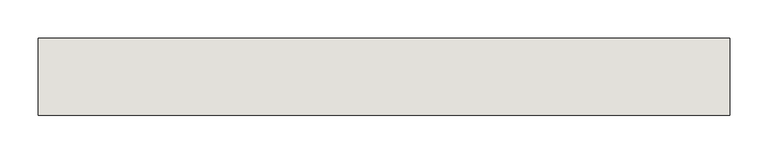
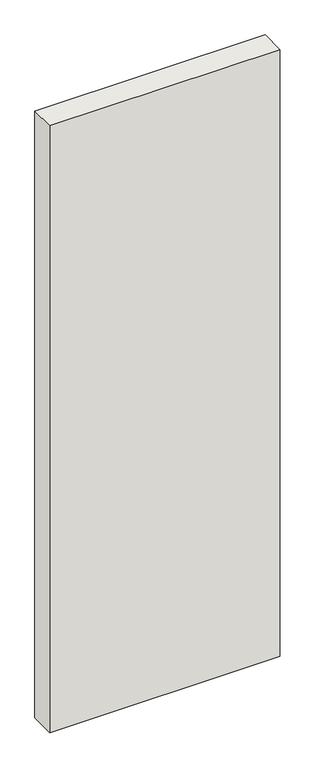
"""IFC4 building model written with IfcOpenShell, lengths in millimetres: wall geometry, Holzwand."""

from ifc_helpers import new_model, si_unit, origin, origin_with_axes, place, context, project, spatial, polyline, outline, extrude, source, transform, mapped, element, save


def wall_35934e9d(model_context):
    return source(origin(), model_context, "Body", "SweptSolid", [
        extrude(outline(polyline([(0.0, 100.0), (900.0, 100.0), (900.0, 0.0), (0.0, 0.0), (0.0, 100.0)])), origin_with_axes(), (0.0, 0.0, 1.0), 2510.0),
    ])


if __name__ == "__main__":
    model = new_model("IFC4")
    model_context = context("Model", 3, world=origin())
    ifc_project = project(units=[si_unit("LENGTHUNIT", "METRE", prefix="MILLI")], contexts=[model_context])
    site = spatial("IfcSite", under=ifc_project)
    building = spatial("IfcBuilding", under=site)
    placement = place(None, origin())
    wall_shape = wall_35934e9d(model_context)
    element("IfcWall", 1, ObjectType="Holzwand", at=placement, inside=building, context=model_context, shape_type="MappedRepresentation", body=[
        mapped(wall_shape, transform((0.0, 0.0, 0.0), x_axis=(1.0, 0.0, 0.0), y_axis=(0.0, 1.0, 0.0), z_axis=(0.0, 0.0, 1.0))),
    ])
    save(model, "model.ifc")

# Revit data of these elements
# Element 1 (IfcWall, "Holzwand")
#   Materials on its faces: "holzschalung"
# Materials
#   "holzschalung": class "Unassigned", colour RGB 128 128 128, transparency 0
